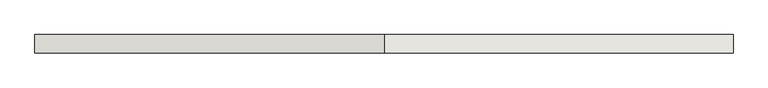
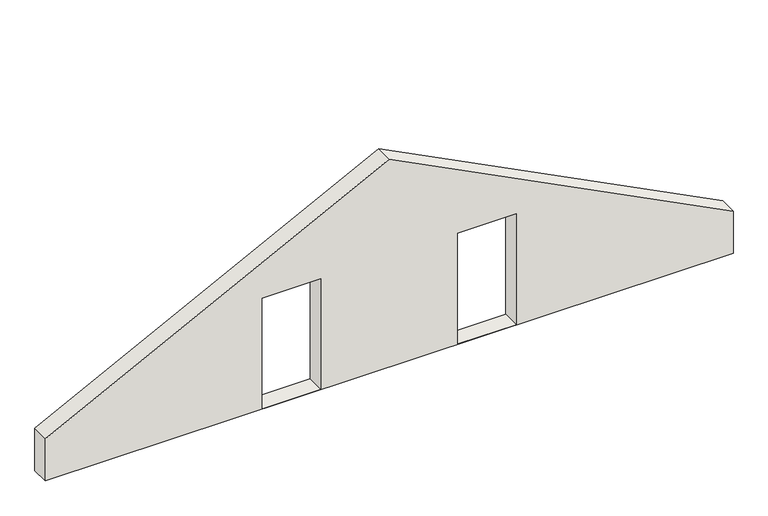
"""IFC4 building model written with IfcOpenShell, lengths in millimetres: wall geometry, 0_3d_modell."""

from ifc_helpers import new_model, si_unit, frame, origin, place, context, project, spatial, polyline, outline, extrude, source, transform, mapped, element, save


def wall_c3aadf07(model_context):
    return source(origin(), model_context, "Body", "SweptSolid", [
        extrude(outline(polyline([(863.3339073, 13300.0), (4251.6781465, 6650.0), (863.3339073, 0.0), (0.0, 0.0), (0.0, 13300.0), (863.3339073, 13300.0)]), holes=[polyline([(10.0, 7975.0), (2270.0, 7975.0), (2270.0, 9110.0), (10.0, 9110.0), (10.0, 7975.0)]), polyline([(10.0, 4190.0), (2270.0, 4190.0), (2270.0, 5325.0), (10.0, 5325.0), (10.0, 4190.0)])]), frame((0.0, 0.0, 0.0), z_axis=(0.0, 1.0, 0.0), x_axis=(0.0, 0.0, 1.0)), (0.0, 0.0, 1.0), 350.0),
    ])


if __name__ == "__main__":
    model = new_model("IFC4")
    model_context = context("Model", 3, world=origin())
    ifc_project = project(units=[si_unit("LENGTHUNIT", "METRE", prefix="MILLI")], contexts=[model_context])
    site = spatial("IfcSite", under=ifc_project)
    building = spatial("IfcBuilding", under=site)
    placement = place(None, origin())
    wall_shape = wall_c3aadf07(model_context)
    element("IfcWall", 1, ObjectType="0_3d_modell", at=placement, inside=building, context=model_context, shape_type="MappedRepresentation", body=[
        mapped(wall_shape, transform((0.0, 0.0, 0.0), x_axis=(1.0, 0.0, 0.0), y_axis=(0.0, 1.0, 0.0), z_axis=(0.0, 0.0, 1.0))),
    ])
    save(model, "model.ifc")

# Revit data of these elements
# Element 1 (IfcWall, "0_3d_modell")
#   Materials on its faces: "holzschalung"
# Materials
#   "holzschalung": class "Unassigned", colour RGB 128 128 128, transparency 0
